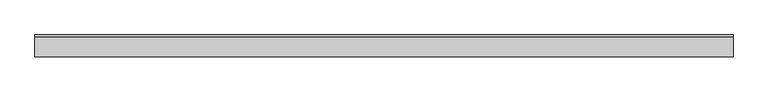
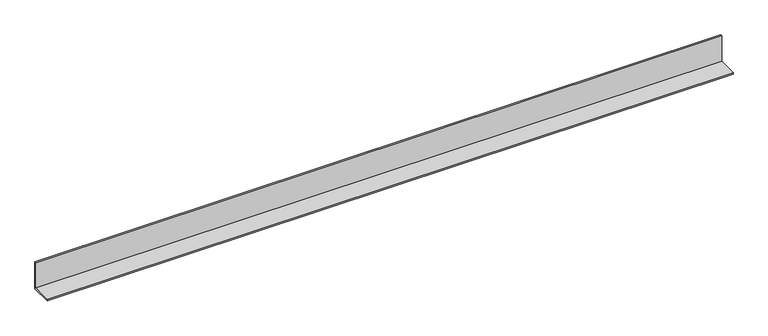
"""IFC4 building model written with IfcOpenShell, lengths in millimetres: proxy geometry, Generic Models 3:Generic Models 1:6:Generic Models 1:6 : Generic Models 3:Generic Models 1:300625:350611:Generic Models 1:6:Generic Models 1:6 : Generic Models 3:Generic Models 1:300625:350611 : Generic Models 3:Generic Models 1:6:Generic Models 1:6 : Generic Models 3:Generic Models 1:300625:350611:3 : Generic Models 3:Generic Models 1:6:Generic Models 1:6 : Generic Models 3:Generic Models 1:300625:350611:Generic Models 1:6:Generic Models 1:6 : Generic Models 3:Generic Models 1:300625:350611 : Generic Models 3:Generic Models 1:6:Generic Models 1:6 : Generic Models 3:Generic Models 1:300625:350611:301824."""

from ifc_helpers import new_model, si_unit, frame, origin, place, context, project, spatial, polyline, outline, extrude, source, transform, mapped, element, save


def generic_models_e8fc80ef(model_context):
    return source(origin(), model_context, "Body", "SweptSolid", [
        extrude(outline(polyline([(-578848.2913841, 0.0), (-578924.4913841, 0.0), (-578924.4913841, 6.35), (-578854.6413841, 6.35), (-578854.6413841, 101.6), (-578848.2913841, 101.6), (-578848.2913841, 0.0)])), frame((599865.8367239, 0.0, 0.0), z_axis=(1.0, 0.0, 0.0), x_axis=(0.0, 1.0, 0.0)), (0.0, 0.0, 1.0), 2438.4),
    ])


if __name__ == "__main__":
    model = new_model("IFC4")
    model_context = context("Model", 3, world=origin())
    ifc_project = project(units=[si_unit("LENGTHUNIT", "METRE", prefix="MILLI")], contexts=[model_context])
    site = spatial("IfcSite", under=ifc_project)
    building = spatial("IfcBuilding", under=site)
    placement = place(None, origin())
    generic_models_shape = generic_models_e8fc80ef(model_context)
    element("IfcBuildingElementProxy", 1, Name="Generic Models 3:Generic Models 1:6:Generic Models 1:6 : Generic Models 3:Generic Models 1:300625:350611:Generic Models 1:6:Generic Models 1:6 : Generic Models 3:Generic Models 1:300625:350611 : Generic Models 3:Generic Models 1:6:Generic Models 1:6 : Generic Models 3:Generic Models 1:300625:350611:3 : Generic Models 3:Generic Models 1:6:Generic Models 1:6 : Generic Models 3:Generic Models 1:300625:350611:Generic Models 1:6:Generic Models 1:6 : Generic Models 3:Generic Models 1:300625:350611 : Generic Models 3:Generic Models 1:6:Generic Models 1:6 : Generic Models 3:Generic Models 1:300625:350611:301824", ObjectType="Generic Models 3:Generic Models 1:6:Generic Models 1:6 : Generic Models 3:Generic Models 1:300625:350611:Generic Models 1:6:Generic Models 1:6 : Generic Models 3:Generic Models 1:300625:350611 : Generic Models 3:Generic Models 1:6:Generic Models 1:6 : Generic Models 3:Generic Models 1:300625:350611:3 : Generic Models 3:Generic Models 1:6:Generic Models 1:6 : Generic Models 3:Generic Models 1:300625:350611:Generic Models 1:6:Generic Models 1:6 : Generic Models 3:Generic Models 1:300625:350611 : Generic Models 3:Generic Models 1:6:Generic Models 1:6 : Generic Models 3:Generic Models 1:300625:350611:301824", at=placement, inside=building, context=model_context, shape_type="MappedRepresentation", body=[
        mapped(generic_models_shape, transform((0.0, 0.0, 0.0), x_axis=(1.0, 0.0, 0.0), y_axis=(0.0, 1.0, 0.0), z_axis=(0.0, 0.0, 1.0))),
    ])
    save(model, "model.ifc")

# Revit data of these elements
# Type "Generic Models 3:Generic Models 1:6:Generic Models 1:6 : Generic Models 3:Generic Models 1:300625:350611:Generic Models 1:6:Generic Models 1:6 : Generic Models 3:Generic Models 1:300625:350611 : Generic Models 3:Generic Models 1:6:Generic Models 1:6 : Generic Models 3:Generic Models 1:300625:350611:3 : Generic Models 3:Generic Models 1:6:Generic Models 1:6 : Generic Models 3:Generic Models 1:300625:350611:Generic Models 1:6:Generic Models 1:6 : Generic Models 3:Generic Models 1:300625:350611 : Generic Models 3:Generic Models 1:6:Generic Models 1:6 : Generic Models 3:Generic Models 1:300625:350611:301824"
#   NameOverride = "Generic Models 3:Generic Models 1:6:Generic Models 1:6 : Generic Models 3:Generic Models 1:300625:350611:Generic Models 1:6:Generic Models 1:6 : Generic Models 3:Generic Models 1:300625:350611 : Generic Models 3:Generic Models 1:6:Generic Models 1:6 : Generic Models 3:Generic Models 1:300625:350611:301824"
#   ObjectTypeOverride = "Generic Models 1:6:Generic Models 1:6 : Generic Models 3:Generic Models 1:300625:350611 : Generic Models 3:Generic Models 1:6:Generic Models 1:6 : Generic Models 3:Generic Models 1:300625:350611"
#   Reference = "Generic Models 1"
#   Tag = "301824"
# Element 1 (IfcBuildingElementProxy, "Generic Models 3:Generic Models 1:6:Generic Models 1:6 : Generic Models 3:Generic Models 1:300625:350611:Generic Models 1:6:Generic Models 1:6 : Generic Models 3:Generic Models 1:300625:350611 : Generic Models 3:Generic Models 1:6:Generic Models 1:6 : Generic Models 3:Generic Models 1:300625:350611:3 : Generic Models 3:Generic Models 1:6:Generic Models 1:6 : Generic Models 3:Generic Models 1:300625:350611:Generic Models 1:6:Generic Models 1:6 : Generic Models 3:Generic Models 1:300625:350611 : Generic Models 3:Generic Models 1:6:Generic Models 1:6 : Generic Models 3:Generic Models 1:300625:350611:301824")
#   Materials on its faces: "6\" Metal Stud Track_1"
# Materials
#   "6\" Metal Stud Track_1": class "Unassigned", colour RGB 120 120 120, transparency 0
